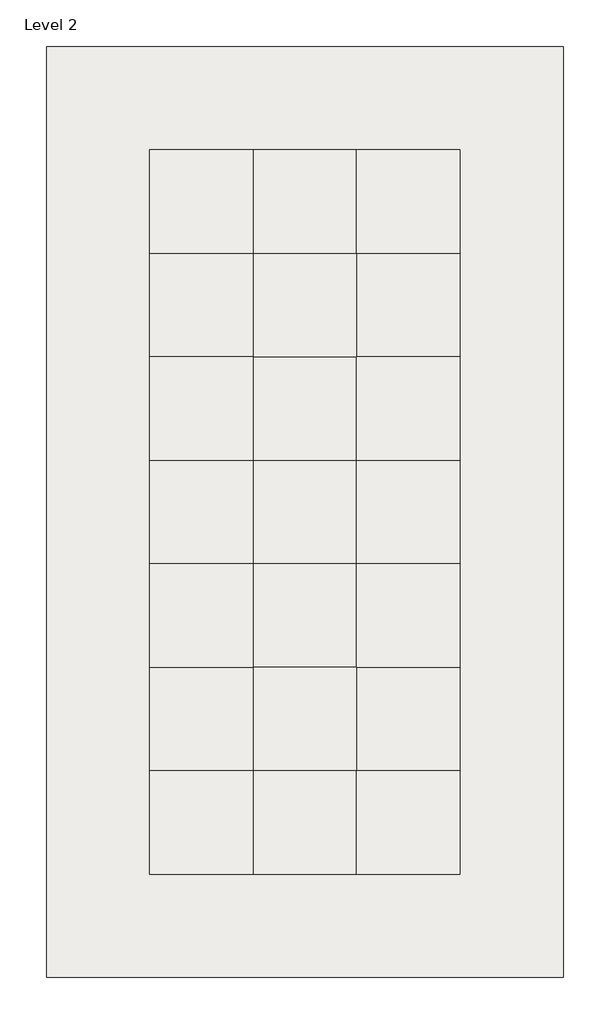
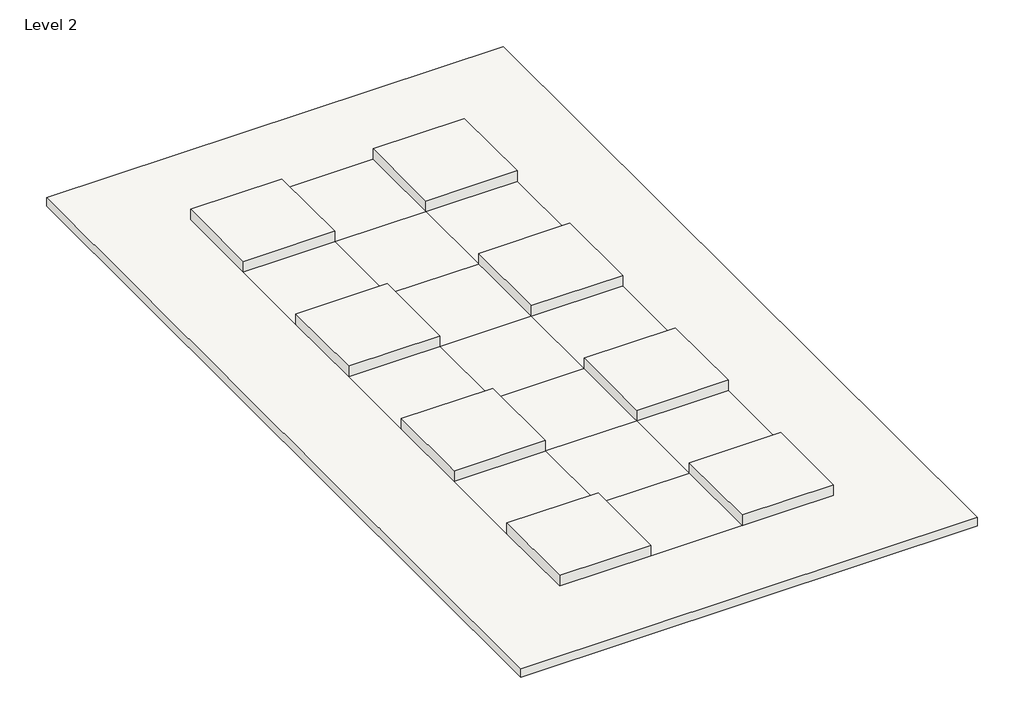
# One storey: 9 roofs.
"""IFC4 building model written with IfcOpenShell, lengths in millimetres."""

from ifc_helpers import new_model, si_unit, origin, place, context, project, spatial, faceted_brep, element, save

model = new_model("IFC4")

# Units and contexts
model_context = context("Model", 3, world=origin())
ifc_project = project(units=[si_unit("LENGTHUNIT", "METRE", prefix="MILLI")], contexts=[model_context])

# Site, building, storey
site = spatial("IfcSite", under=ifc_project)
building = spatial("IfcBuilding", under=site)
storey = spatial("IfcBuildingStorey", under=building, Name="Level 2", Elevation=8000.0)

# Roofs
placement = place(None, origin())
element("IfcRoof", 1, ObjectType="Bauder_RoofCoveringSystem_ExtensiveGreenRoofSystem_WildflowerBlanket", at=placement, inside=storey, context=model_context, shape_type="Brep", body=[
    faceted_brep([(-674.7340554, 1676.2074539, 8000.0), (1325.2659446, 1676.2074539, 8000.0), (1325.2659446, -323.7925461, 8000.0), (-674.7340554, -323.7925461, 8000.0), (1325.2659446, 1676.2074539, 8445.0), (-674.7340554, 1676.2074539, 8445.0), (-674.7340554, -323.7925461, 8445.0), (1325.2659446, -323.7925461, 8445.0), (1325.2659446, 1676.2074539, 8200.0), (-674.7340554, 1676.2074539, 8200.0), (-674.7340554, -323.7925461, 8200.0), (1325.2659446, -323.7925461, 8200.0)], [[[0, 1, 2, 3]], [[4, 5, 6, 7]], [[5, 4, 8, 1, 0, 9]], [[6, 5, 9, 0, 3, 10]], [[7, 6, 10, 3, 2, 11]], [[4, 7, 11, 2, 1, 8]]]),
])
element("IfcRoof", 2, ObjectType="Bauder_RoofCoveringSystem_ExtensiveGreenRoofSystem_WildflowerBlanket", at=placement, inside=storey, context=model_context, shape_type="Brep", body=[
    faceted_brep([(3325.2659446, 1676.2074539, 8000.0), (5325.2659446, 1676.2074539, 8000.0), (5325.2659446, -323.7925461, 8000.0), (3325.2659446, -323.7925461, 8000.0), (5325.2659446, 1676.2074539, 8445.0), (3325.2659446, 1676.2074539, 8445.0), (3325.2659446, -323.7925461, 8445.0), (5325.2659446, -323.7925461, 8445.0), (5325.2659446, 1676.2074539, 8200.0), (3325.2659446, 1676.2074539, 8200.0), (3325.2659446, -323.7925461, 8200.0), (5325.2659446, -323.7925461, 8200.0)], [[[0, 1, 2, 3]], [[4, 5, 6, 7]], [[5, 4, 8, 1, 0, 9]], [[6, 5, 9, 0, 3, 10]], [[7, 6, 10, 3, 2, 11]], [[4, 7, 11, 2, 1, 8]]]),
])
element("IfcRoof", 3, ObjectType="Bauder_RoofCoveringSystem_ExtensiveGreenRoofSystem_WildflowerBlanket", at=placement, inside=storey, context=model_context, shape_type="Brep", body=[
    faceted_brep([(3325.2659446, -2323.7925461, 8000.0), (5325.2659446, -2323.7925461, 8000.0), (5325.2659446, -4323.7925461, 8000.0), (3325.2659446, -4323.7925461, 8000.0), (5325.2659446, -2323.7925461, 8445.0), (3325.2659446, -2323.7925461, 8445.0), (3325.2659446, -4323.7925461, 8445.0), (5325.2659446, -4323.7925461, 8445.0), (5325.2659446, -2323.7925461, 8200.0), (3325.2659446, -2323.7925461, 8200.0), (3325.2659446, -4323.7925461, 8200.0), (5325.2659446, -4323.7925461, 8200.0)], [[[0, 1, 2, 3]], [[4, 5, 6, 7]], [[5, 4, 8, 1, 0, 9]], [[6, 5, 9, 0, 3, 10]], [[7, 6, 10, 3, 2, 11]], [[4, 7, 11, 2, 1, 8]]]),
])
element("IfcRoof", 4, ObjectType="Bauder_RoofCoveringSystem_ExtensiveGreenRoofSystem_WildflowerBlanket", at=placement, inside=storey, context=model_context, shape_type="Brep", body=[
    faceted_brep([(3325.2659446, -6323.7925461, 8000.0), (5325.2659446, -6323.7925461, 8000.0), (5325.2659446, -8323.7925461, 8000.0), (3325.2659446, -8323.7925461, 8000.0), (5325.2659446, -6323.7925461, 8445.0), (3325.2659446, -6323.7925461, 8445.0), (3325.2659446, -8323.7925461, 8445.0), (5325.2659446, -8323.7925461, 8445.0), (5325.2659446, -6323.7925461, 8200.0), (3325.2659446, -6323.7925461, 8200.0), (3325.2659446, -8323.7925461, 8200.0), (5325.2659446, -8323.7925461, 8200.0)], [[[0, 1, 2, 3]], [[4, 5, 6, 7]], [[5, 4, 8, 1, 0, 9]], [[6, 5, 9, 0, 3, 10]], [[7, 6, 10, 3, 2, 11]], [[4, 7, 11, 2, 1, 8]]]),
])
element("IfcRoof", 5, ObjectType="Bauder_RoofCoveringSystem_ExtensiveGreenRoofSystem_WildflowerBlanket", at=placement, inside=storey, context=model_context, shape_type="Brep", body=[
    faceted_brep([(3325.2659446, -10323.7925461, 8000.0), (5325.2659446, -10323.7925461, 8000.0), (5325.2659446, -12323.7925461, 8000.0), (3325.2659446, -12323.7925461, 8000.0), (5325.2659446, -10323.7925461, 8445.0), (3325.2659446, -10323.7925461, 8445.0), (3325.2659446, -12323.7925461, 8445.0), (5325.2659446, -12323.7925461, 8445.0), (5325.2659446, -10323.7925461, 8200.0), (3325.2659446, -10323.7925461, 8200.0), (3325.2659446, -12323.7925461, 8200.0), (5325.2659446, -12323.7925461, 8200.0)], [[[0, 1, 2, 3]], [[4, 5, 6, 7]], [[5, 4, 8, 1, 0, 9]], [[6, 5, 9, 0, 3, 10]], [[7, 6, 10, 3, 2, 11]], [[4, 7, 11, 2, 1, 8]]]),
])
element("IfcRoof", 6, ObjectType="Bauder_RoofCoveringSystem_ExtensiveGreenRoofSystem_WildflowerBlanket", at=placement, inside=storey, context=model_context, shape_type="Brep", body=[
    faceted_brep([(-674.7340554, -10323.7925461, 8000.0), (1325.2659446, -10323.7925461, 8000.0), (1325.2659446, -12323.7925461, 8000.0), (-674.7340554, -12323.7925461, 8000.0), (1325.2659446, -10323.7925461, 8445.0), (-674.7340554, -10323.7925461, 8445.0), (-674.7340554, -12323.7925461, 8445.0), (1325.2659446, -12323.7925461, 8445.0), (1325.2659446, -10323.7925461, 8200.0), (-674.7340554, -10323.7925461, 8200.0), (-674.7340554, -12323.7925461, 8200.0), (1325.2659446, -12323.7925461, 8200.0)], [[[0, 1, 2, 3]], [[4, 5, 6, 7]], [[5, 4, 8, 1, 0, 9]], [[6, 5, 9, 0, 3, 10]], [[7, 6, 10, 3, 2, 11]], [[4, 7, 11, 2, 1, 8]]]),
])
element("IfcRoof", 7, ObjectType="Bauder_RoofCoveringSystem_ExtensiveGreenRoofSystem_WildflowerBlanket", at=placement, inside=storey, context=model_context, shape_type="Brep", body=[
    faceted_brep([(-674.7340554, -6323.7925461, 8000.0), (1325.2659446, -6323.7925461, 8000.0), (1325.2659446, -8323.7925461, 8000.0), (-674.7340554, -8323.7925461, 8000.0), (1325.2659446, -6323.7925461, 8445.0), (-674.7340554, -6323.7925461, 8445.0), (-674.7340554, -8323.7925461, 8445.0), (1325.2659446, -8323.7925461, 8445.0), (1325.2659446, -6323.7925461, 8200.0), (-674.7340554, -6323.7925461, 8200.0), (-674.7340554, -8323.7925461, 8200.0), (1325.2659446, -8323.7925461, 8200.0)], [[[0, 1, 2, 3]], [[4, 5, 6, 7]], [[5, 4, 8, 1, 0, 9]], [[6, 5, 9, 0, 3, 10]], [[7, 6, 10, 3, 2, 11]], [[4, 7, 11, 2, 1, 8]]]),
])
element("IfcRoof", 8, ObjectType="Bauder_RoofCoveringSystem_ExtensiveGreenRoofSystem_WildflowerBlanket", at=placement, inside=storey, context=model_context, shape_type="Brep", body=[
    faceted_brep([(-674.7340554, -2323.7925461, 8000.0), (1325.2659446, -2323.7925461, 8000.0), (1325.2659446, -4323.7925461, 8000.0), (-674.7340554, -4323.7925461, 8000.0), (1325.2659446, -2323.7925461, 8445.0), (-674.7340554, -2323.7925461, 8445.0), (-674.7340554, -4323.7925461, 8445.0), (1325.2659446, -4323.7925461, 8445.0), (1325.2659446, -2323.7925461, 8200.0), (-674.7340554, -2323.7925461, 8200.0), (-674.7340554, -4323.7925461, 8200.0), (1325.2659446, -4323.7925461, 8200.0)], [[[0, 1, 2, 3]], [[4, 5, 6, 7]], [[5, 4, 8, 1, 0, 9]], [[6, 5, 9, 0, 3, 10]], [[7, 6, 10, 3, 2, 11]], [[4, 7, 11, 2, 1, 8]]]),
])
element("IfcRoof", 9, ObjectType="Roof_Concrete-200mm", at=placement, inside=storey, context=model_context, shape_type="Brep", body=[
    faceted_brep([(-2674.7340554, -14323.7925461, 8200.0), (-2674.7340554, -14323.7925461, 8000.0), (7325.2659446, -14323.7925461, 8000.0), (7325.2659446, -14323.7925461, 8200.0), (-2674.7340554, 3676.2074539, 8200.0), (-2674.7340554, 3676.2074539, 8000.0), (7325.2659446, 3676.2074539, 8200.0), (7325.2659446, 3676.2074539, 8000.0), (3325.2659446, 1676.2074539, 8200.0), (1325.2659446, 1676.2074539, 8200.0), (1325.2659446, -323.7925461, 8200.0), (3325.2659446, -323.7925461, 8200.0), (1325.2659446, 1676.2074539, 8000.0), (3325.2659446, 1676.2074539, 8000.0), (3325.2659446, -323.7925461, 8000.0), (1325.2659446, -323.7925461, 8000.0), (1325.2659446, -2323.7925461, 8200.0), (-674.7340554, -323.7925461, 8200.0), (-674.7340554, -2323.7925461, 8200.0), (3325.2659446, -2323.7925461, 8200.0), (5325.2659446, -2323.7925461, 8200.0), (5325.2659446, -323.7925461, 8200.0), (-674.7340554, -2323.7925461, 8000.0), (-674.7340554, -323.7925461, 8000.0), (1325.2659446, -2323.7925461, 8000.0), (3325.2659446, -2323.7925461, 8000.0), (5325.2659446, -323.7925461, 8000.0), (5325.2659446, -2323.7925461, 8000.0), (1325.2659446, -4323.7925461, 8200.0), (3325.2659446, -4323.7925461, 8200.0), (3325.2659446, -4323.7925461, 8000.0), (1325.2659446, -4323.7925461, 8000.0), (1325.2659446, -6323.7925461, 8200.0), (-674.7340554, -4323.7925461, 8200.0), (-674.7340554, -6323.7925461, 8200.0), (5325.2659446, -6323.7925461, 8200.0), (5325.2659446, -4323.7925461, 8200.0), (3325.2659446, -6323.7925461, 8200.0), (-674.7340554, -6323.7925461, 8000.0), (-674.7340554, -4323.7925461, 8000.0), (1325.2659446, -6323.7925461, 8000.0), (3325.2659446, -6323.7925461, 8000.0), (5325.2659446, -4323.7925461, 8000.0), (5325.2659446, -6323.7925461, 8000.0), (1325.2659446, -12323.7925461, 8200.0), (3325.2659446, -12323.7925461, 8200.0), (3325.2659446, -10323.7925461, 8200.0), (1325.2659446, -10323.7925461, 8200.0), (3325.2659446, -12323.7925461, 8000.0), (1325.2659446, -12323.7925461, 8000.0), (1325.2659446, -10323.7925461, 8000.0), (3325.2659446, -10323.7925461, 8000.0), (1325.2659446, -8323.7925461, 8200.0), (-674.7340554, -8323.7925461, 8200.0), (-674.7340554, -10323.7925461, 8200.0), (3325.2659446, -8323.7925461, 8200.0), (5325.2659446, -10323.7925461, 8200.0), (5325.2659446, -8323.7925461, 8200.0), (-674.7340554, -10323.7925461, 8000.0), (-674.7340554, -8323.7925461, 8000.0), (1325.2659446, -8323.7925461, 8000.0), (3325.2659446, -8323.7925461, 8000.0), (5325.2659446, -8323.7925461, 8000.0), (5325.2659446, -10323.7925461, 8000.0), (-674.7340554, 1676.2074539, 8000.0), (-674.7340554, 1676.2074539, 8200.0), (5325.2659446, 1676.2074539, 8200.0), (5325.2659446, 1676.2074539, 8000.0), (5325.2659446, -12323.7925461, 8000.0), (5325.2659446, -12323.7925461, 8200.0), (-674.7340554, -12323.7925461, 8000.0), (-674.7340554, -12323.7925461, 8200.0)], [[[0, 1, 2, 3]], [[1, 0, 4, 5]], [[6, 7, 5, 4]], [[3, 2, 7, 6]], [[8, 9, 10, 11]], [[12, 13, 14, 15]], [[16, 10, 17, 18]], [[11, 10, 16, 19]], [[20, 21, 11, 19]], [[22, 23, 15, 24]], [[15, 14, 25, 24]], [[25, 14, 26, 27]], [[19, 16, 28, 29]], [[24, 25, 30, 31]], [[32, 28, 33, 34]], [[35, 36, 29, 37]], [[38, 39, 31, 40]], [[41, 30, 42, 43]], [[44, 45, 46, 47]], [[48, 49, 50, 51]], [[47, 52, 53, 54]], [[47, 46, 55, 52]], [[56, 57, 55, 46]], [[58, 59, 60, 50]], [[51, 50, 60, 61]], [[51, 61, 62, 63]], [[52, 55, 37, 32]], [[29, 28, 32, 37]], [[61, 60, 40, 41]], [[31, 30, 41, 40]], [[9, 12, 15, 10]], [[10, 15, 23, 17]], [[17, 23, 64, 65]], [[12, 9, 65, 64]], [[66, 67, 26, 21]], [[21, 26, 14, 11]], [[11, 14, 13, 8]], [[67, 66, 8, 13]], [[20, 27, 42, 36]], [[36, 42, 30, 29]], [[29, 30, 25, 19]], [[27, 20, 19, 25]], [[16, 24, 31, 28]], [[28, 31, 39, 33]], [[33, 39, 22, 18]], [[24, 16, 18, 22]], [[32, 40, 60, 52]], [[52, 60, 59, 53]], [[53, 59, 38, 34]], [[40, 32, 34, 38]], [[35, 43, 62, 57]], [[57, 62, 61, 55]], [[55, 61, 41, 37]], [[43, 35, 37, 41]], [[56, 63, 68, 69]], [[69, 68, 48, 45]], [[45, 48, 51, 46]], [[63, 56, 46, 51]], [[47, 50, 49, 44]], [[44, 49, 70, 71]], [[71, 70, 58, 54]], [[50, 47, 54, 58]], [[4, 0, 3, 6], [9, 8, 66, 21, 20, 36, 35, 57, 56, 69, 45, 44, 71, 54, 53, 34, 33, 18, 17, 65]], [[7, 2, 1, 5], [13, 12, 64, 23, 22, 39, 38, 59, 58, 70, 49, 48, 68, 63, 62, 43, 42, 27, 26, 67]]]),
])

save(model, "model.ifc")

# Revit data of these elements
# Type "Bauder_RoofCoveringSystem_ExtensiveGreenRoofSystem_WildflowerBlanket"
#   Keynote = "Q37"
#   Type IFC Predefined Type = "FLAT_ROOF"
#   Export Type to IFC As = "IfcRoofType"
#   Model = "Bauder Biodiverse Wildflower Blanket - Extensive Green Roof System"
#   Manufacturer = "Bauder Ltd"
#   Type Comments = "Wildflower Blanket"
#   URL = "https://www.bauder.co.uk/"
#   Description = "Bauder Biodiverse GreenRoof system incorporating WB 25 mm UK Native Species Wildflower Blanket with Biodiverse Substrate, Filter Fleece, DSE40 Polyethylene Drainage and Protection Layer, and FSM600 Polyester-Polypropylene fibre protection mat."
#   Assembly Code = "B3010"
#   NBSDescription = "Extensive green roof system"
#   NBSReference = "45-40-47/130"
#   BIMObjectName = "Bauder_RoofCoveringSystem_ExtensiveGreenRoofSystem_WildflowerBlanket"
#   AccessibilityPerformance = "n/a"
#   CodePerformance = "n/a"
#   Color = "n/a"
#   Constituents = "n/a"
#   DurationUnit = "Year"
#   ExpectedLife = "n/a"
#   Features = "This BIM Object must be supported by a project specific specification from Bauder, incorporating system build-up, detail design and performance calculations if a full Bauder system guarantee is required. Please contact your local Bauder Representative or technical@bauder.co.uk"
#   Finish = "n/a"
#   Grade = "n/a"
#   Material = "n/a"
#   ModelReference = "Bauder Biodiverse Wildflower Blanket - Extensive Green Roof System"
#   Name = "RoofCoveringSystem_Bauder_ExtensiveGreenRoofSystem"
#   ReplacementCost = "n/a"
#   Shape = "n/a"
#   Size = "n/a"
#   SustainabilityPerformance = "Bauder Germany ISO14001: Certificate No.: 70499/03-15 e, Bauder UK ISO14001:Certificate No. 19ACM6595R, EN1271, BREEAM Credits Available"
#   WarrantyDescription = "Guarantee options could include ‘Product’, ‘Product and Workmanship’ and ‘Product, Workmanship and Design’ Guarantees. All guarantees available for this system are subject to the works being carried out in accordance with the Bauder specification and being installed by a Bauder Approved installer. For full details and further information regarding guarantees and alternative systems please contact your local Bauder Representative or technical@bauder.co.uk"
#   WarrantyDurationLabor = "n/a"
#   WarrantyDurationParts = "n/a"
#   WarrantyDurationUnit = "Year"
#   WarrantyGuarantorLabor = "n/a"
#   WarrantyGuarantorParts = "technical@bauder.co.uk"
#   Certification = "Comply with GRO Green Roof Code of Practice and FLL Standards"
#   EdgeRestraints = "Perforated edge trim where required, refer to Bauder Project Specific Specification"
#   MoistureControlDrainageAncillaries = "n/a"
#   MoistureControlDrainageLayer = "Bauder DSE40 40 mm Polyethylene Drainage and Protection Layer"
#   MoistureControlFilterMembrane = "Bauder Filter Fleece 1 mm Polypropylene Filter Fleece"
#   MoistureControlMoistureRetentionMat = "Polypropylene mesh bonded to a moisture permeable base carrier sheet integral to the Blanket"
#   PlantingSystemsAntierosionMat = "Jute Net where exposed, refer to Bauder Project Specific Specification"
#   PlantingSystemsPlantingMedium = "Bauder Biodiverse Substrate Recycled crushed brick, expanded clay shale and composted pine bark"
#   PlantingSystemsVegetation = "Bauder WB 25 mm UK Native Species Wildflower Blanket"
#   PlantingSystemsVegetationBarrier = "20-40 mm Rounded-Washed Stones, refer to Bauder Project Specific Specification"
#   ProjectSpecificationAndDesign = "This BIM Object must be supported by a project specific specification from Bauder, incorporating system build-up, detail design and performance calculations if a full Bauder system warranty is required. Please contact your local Bauder Representative or technical@bauder.co.uk"
#   ProtectionProtectionLayer = "Bauder FSM600 4 mm Polyester-Polypropylene fibre protection mat"
#   ProtectionRootBarrier = "As per project specific Bauder Specification"
#   ProtectionSeparationLayer = "n/a"
#   SystemManufacturer = "Bauder Ltd"
#   WarrantyConsiderations = "All guarantees available for this system are subject to the works being carried out in accordance with the Bauder specification and being installed by a Bauder Approved installer. For full details and further information regarding guarantees and alternative systems please contact your local Bauder Representative or technical@bauder.co.uk"
#   Update = "1900-12-31T23:59:59"
#   Documentation = "https://www.bauder.co.uk/technical-centre/technical-literature/system-brochures"
#   DocumentReference = "http://www.bauder.co.uk/"
#   IfcExportAs = "IfcRoofType"
#   IfcExportType = "FLAT_ROOF"
#   MethodOfMesurement = "n/a"
#   Process = "Replacement at service life intervals"
#   FireRating = "n/a"
#   _Author = "AM"
#   _AuthorizedBy = "bimstore"
#   _CreatedBy = "technical@bauder.co.uk"
#   _DistributedBy = "www.bimstore.co"
#   AssetType = "Fixed"
#   ClassificationName = "Uniclass2015"
#   ClassificationValue = "Ss_45_40_47_09"
#   CreatedBy = "technical@bauder.co.uk"
#   CreatedOn = "2023-02-10 T00:00:00"
#   DocumentationCertificates = "n/a"
#   DocumentationInstallationGuide = "https://www.bauder.co.uk/technical-centre"
#   DocumentationLiterature = "https://www.bauder.co.uk/technical-centre"
#   DocumentationMaintenance = "https://www.bauder.co.uk/technical-centre/maintenance-advice"
#   DocumentationTechnical = "https://www.bauder.co.uk/green-roofs/extensive-green-roofs/biodiverse-or-brown-roofs/wildflower-blanket"
#   ManufacturerName = "Bauder Ltd"
#   ModelNumber = "0905_WB-BioS-FF-D4-F6"
#   ProductionYear = "2017"
#   ReferencedStandard = "n/a"
#   SpareParts = "n/a"
#   TypeName = "Wildflower Blanket"
#   NBSNote = "n/a"
#   NBSObjectName = "Bauder - Extensive green roof system"
#   NBSOfficeMasterTag = "n/a"
#   Ballast = "n/a"
#   CarrierMembraneFixing = "n/a"
#   CarrierMembraneType = "n/a"
#   FillToPerimeterUpstands = "n/a"
#   FilterLayer = "n/a"
#   InsulationFixing = "n/a"
#   InsulationType = "n/a"
#   LiquidAppliedWaterproofCoatingReinforcement = "n/a"
#   LiquidAppliedWaterproofCoatingSurfaceTreatment = "n/a"
#   LiquidAppliedWaterproofCoatingType = "n/a"
#   PreparationExistingSubstrates = "n/a"
#   PreparationHorizontalWork = "n/a"
#   PreparationSkirtingsAndVerticalWork = "n/a"
#   ProtectionLayer = "n/a"
#   SystemAccessories = "n/a"
#   WaterproofCoveringFirstLayerAttachment = "n/a"
#   WaterproofCoveringFirstLayerType = "n/a"
#   WaterproofCoveringIntermediateLayerAttachment = "n/a"
#   WaterproofCoveringIntermediateLayerType = "n/a"
#   WaterproofCoveringTopLayerAttachment = "n/a"
#   InsulationAttachment = "n/a"
#   IsolatingLayer = "n/a"
#   CarrierMembraneAttachment = "n/a"
#   LiquidAppliedWaterproofCoatingWearingCourse = "n/a"
#   VapourControlLayer = "n/a"
#   VapourControlLayerAttachment_Bauder = "n/a"
#   WaterproofCoveringJoints = "n/a"
#   WaterproofCoveringType = "n/a"
#   SeparatingLayer = "n/a"
#   WaterproofCoveringAccessories = "Yes"
#   WaterproofCoveringAttachment = "n/a"
#   UpperProtectionLayer = "n/a"
#   LowerProtectionLayer = "n/a"
#   WaterproofCoveringTopLayerType = "n/a"
#   DetailWorkAncillaryItems = "Detail as per project specific Bauder Specification"
#   DetailWorkCoverStrips = "Detail as per project specific Bauder Specification"
#   DetailWorkFlashings = "Detail as per project specific Bauder Specification"
#   DetailWorkSkirtingsAndUpstands = "Detail as per project specific Bauder Specification"
#   DetailWorkWeltedDrips = "Detail as per project specific Bauder Specification"
#   OverlayFixing = "n/a"
#   OverlayType = "n/a"
#   SurfaceProtection = "n/a"
#   VapourControlLayerAttachment = "n/a"
#   VapourControlLayerType = "n/a"
#   Cost = 0
#   NominalHeight = 0 mm
#   NominalLength = 0 mm
#   TotalArea = 0 m²
#   NominalDepth = 0 mm
#   IsExternal = yes
#   _BimSpecGuid = 0
#   _BSBibleVersion = 16
#   _CurrentRevision = 4
#   Layers, outside or top first: 100 mm "Bauder_Vegetation_BauderGREEN-WB-Wildflower-Blanket" (function 5); 100 mm "Bauder_ExtensiveSubstrate_BauderGREEN-SUB-BM-UK" (function 2); 1 mm "Bauder_FilterFleece_BauderGREEN-FV-125-100" (function 3); 40 mm "Bauder_DrainageBoard_BauderGREEN-DSE-40" (function 3); 4 mm "Bauder_ProtectionMat_BauderGREEN-FSM-600" (function 3); 200 mm "Concrete" (function 1)
# Type "Roof_Concrete-200mm"
#   Layers, outside or top first: 200 mm "Concrete" (function 1)
# Elements 1, 2, 3, 4, 5, 6, 7, 8 (IfcRoof, "Bauder_RoofCoveringSystem_ExtensiveGreenRoofSystem_WildflowerBlanket")
#   built-in parameter 1001705 = 27.7067 (stored number, unit not read)
#   built-in parameter 1001710 = 33615
#   Phase Created = New Construction
#   Materials on its faces: "Concrete", "Bauder_Vegetation_BauderGREEN-WB-Wildflower-Blanket"
# Element 9 (IfcRoof, "Roof_Concrete-200mm")
#   built-in parameter 1001710 = 33615
#   Phase Created = New Construction
#   Materials on its faces: "Concrete"
# Materials
#   "Bauder_Vegetation_BauderGREEN-WB-Wildflower-Blanket": class "Unassigned", colour RGB 71 83 38, transparency 0, Mtrl_Author = "AM", Mtrl_AuthorizedBy = "bimstore", Mtrl_DistributedBy = "www.bimstore.co", Mtrl_AccessibilityPerformance = "n/a", Mtrl_AssetIdentifier = "Please record on commissioning", Mtrl_AssetType = "Fixed", Mtrl_BarCode = "Please record on commissioning", Mtrl_ClassificationName = "Uniclass2020", Mtrl_ClassificationValue = "Ss_45_40_47_09", Mtrl_CodePerformance = "n/a", Mtrl_Color = "n/a", Mtrl_Constituents = "n/a", Mtrl_CreatedBy = "technical@bauder.co.uk", Mtrl_CreatedOn = "2023-02-10 T00:00:00", Mtrl_DocumentationCertificates = "https://www.bimstore.co/products/extensive-green-roof-system-wildflower-blanket/document/product-certificates", Mtrl_DocumentationInstallationGuide = "https://www.bimstore.co/products/extensive-green-roof-system-wildflower-blanket/document/installation-guide", Mtrl_DocumentationLiterature = "https://www.bimstore.co/products/extensive-green-roof-system-wildflower-blanket/document/product-literature", Mtrl_DocumentationMaintenance = "https://www.bimstore.co/products/extensive-green-roof-system-wildflower-blanket/document/maintenance-information", Mtrl_DocumentationTechnical = "https://www.bimstore.co/products/extensive-green-roof-system-wildflower-blanket/document/technical-data-sheet", Mtrl_DurationUnit = "Year", Mtrl_Features = "n/a", Mtrl_Finish = "n/a", Mtrl_Grade = "n/a", Mtrl_InstallationDate = "Please record on commissioning", Mtrl_ManufacturerName = "Bauder Ltd", Mtrl_Material = "Substrate and wildflower plants, embedded in a nylon mesh, with a moisture retention fleece", Mtrl_ModelNumber = "BauderGREEN-WB-Wildflower-Blanket", Mtrl_ModelReference = "Vegetation", Mtrl_ProductionYear = "2023", Mtrl_ReferencedStandard = "n/a", Mtrl_Shape = "n/a", Mtrl_Size = "n/a", Mtrl_SpareParts = "n/a", Mtrl_TypeName = "BauderGREEN-WB-Wildflower-Blanket", Mtrl_WarrantyDescription = "As part of Bauder system guarantee, per specification", Mtrl_WarrantyDurationUnit = "Year", Mtrl_WarrantyGuarantorLabor = "technical@bauder.co.uk", Mtrl_WarrantyGuarantorParts = "technical@bauder.co.uk", Mtrl_WarrantyStartDate = "Please record on commissioning", Mtrl_IfcExportAs = "IfcRoofType", Mtrl_IfcExportType = "FLAT_ROOF", Mtrl_BIMObjectName = "Bauder_Vegetation_BauderGREEN-WB-Wildflower-Blanket", Mtrl_NBSDescription = "n/a", Mtrl_NBSNote = "n/a", Mtrl_NBSObjectName = "n/a", Mtrl_NBSOfficeMasterTag = "n/a", Mtrl_NBSReference = "Q37", Mtrl_Ballast = "n/a", Mtrl_CarrierMembraneAttachment = "n/a", Mtrl_CarrierMembraneFixing = "n/a", Mtrl_CarrierMembraneType = "n/a", Mtrl_Certification = "Comply with GRO Green Roof Code of Practice and FLL Standards", Mtrl_DetailWorkAncillaryItems = "Detail as per project specific Bauder Specification", Mtrl_DetailWorkCoverStrips = "Detail as per project specific Bauder Specification", Mtrl_DetailWorkFlashings = "Detail as per project specific Bauder Specification", Mtrl_DetailWorkSkirtingsAndUpstands = "Detail as per project specific Bauder Specification", Mtrl_DetailWorkWeltedDrips = "Detail as per project specific Bauder Specification", Mtrl_EdgeRestraints = "Detail as per project specific Bauder Specification", Mtrl_FillToPerimeterUpstands = "n/a", Mtrl_FilterLayer = "n/a", Mtrl_InsulationAttachment = "As per project specific Bauder Specification", Mtrl_InsulationFixing = "As per project specific Bauder Specification", Mtrl_InsulationType = "As per project specific Bauder Specification", Mtrl_IsolatingLayer = "n/a", Mtrl_LiquidAppliedWaterproofCoatingReinforcement = "As per project specific Bauder Specification", Mtrl_LiquidAppliedWaterproofCoatingSurfaceTreatment = "As per project specific Bauder Specification", Mtrl_LiquidAppliedWaterproofCoatingType = "As per project specific Bauder Specification", Mtrl_LiquidAppliedWaterproofCoatingWearingCourse = "As per project specific Bauder Specification", Mtrl_LowerProtectionLayer = "n/a", Mtrl_MoistureControlDrainageAncillaries = "n/a", Mtrl_MoistureControlDrainageLayer = "n/a", Mtrl_MoistureControlFilterMembrane = "n/a", Mtrl_MoistureControlMoistureRetentionMat = "n/a", Mtrl_OverlayFixing = "n/a", Mtrl_OverlayType = "n/a", Mtrl_PlantingSystemsAntierosionMat = "n/a", Mtrl_PlantingSystemsPlantingMedium = "As per project specific Bauder Specification", Mtrl_PlantingSystemsVegetation = "As per project specific Bauder Specification", Mtrl_PlantingSystemsVegetationBarrier = "As per project specific Bauder Specification", Mtrl_PreparationExistingSubstrates = "n/a", Mtrl_PreparationHorizontalWork = "n/a", Mtrl_PreparationSkirtingsAndVerticalWork = "n/a", Mtrl_ProjectSpecificationAndDesign = "This BIM Object must be supported by a project specific specification from Bauder, incorporating system build-up, detail design and performance calculations if a full Bauder system warranty is required. Please contact your local Bauder Representative or technical@bauder.co.uk", Mtrl_ProtectionLayer = "n/a", Mtrl_ProtectionProtectionLayer = "n/a", Mtrl_ProtectionRootBarrier = "As per project specific Bauder Specification", Mtrl_ProtectionSeparationLayer = "n/a", Mtrl_SeparatingLayer = "n/a", Mtrl_SurfaceProtection = "n/a", Mtrl_SystemAccessories = "n/a", Mtrl_SystemManufacturer = "Bauder Ltd", Mtrl_Update = "1900-12-31 T23:59:59", Mtrl_UpperProtectionLayer = "n/a", Mtrl_VapourControlLayerAttachment = "As per project specific Bauder Specification", Mtrl_VapourControlLayerAttachment_Bauder = "As per project specific Bauder Specification", Mtrl_VapourControlLayerType = "As per project specific Bauder Specification", Mtrl_WarrantyConsiderations = "All guarantees available for this system are subject to the works being carried out in accordance with the Bauder specification and being installed by a Bauder Approved installer. For full details and further information regarding guarantees and alternative systems please contact your local Bauder Representative or technical@bauder.co.uk", Mtrl_WaterproofCoveringAccessories = "As per project specific Bauder Specification", Mtrl_WaterproofCoveringAttachment = "As per project specific Bauder Specification", Mtrl_WaterproofCoveringFirstLayerAttachment = "As per project specific Bauder Specification", Mtrl_WaterproofCoveringFirstLayerType = "As per project specific Bauder Specification", Mtrl_WaterproofCoveringIntermediateLayerAttachment = "As per project specific Bauder Specification", Mtrl_WaterproofCoveringIntermediateLayerType = "As per project specific Bauder Specification", Mtrl_WaterproofCoveringJoints = "As per project specific Bauder Specification", Mtrl_WaterproofCoveringTopLayerAttachment = "As per project specific Bauder Specification", Mtrl_WaterproofCoveringTopLayerType = "As per project specific Bauder Specification", Mtrl_WaterproofCoveringType = "As per project specific Bauder Specification", Cost = 0, Mtrl_ReplacementCost = 0, Mtrl_NominalDepth = 30 mm, Mtrl_NominalHeight = 0 mm, Mtrl_NominalLength = 0 mm, Mtrl_BimSpecGuid = 0, Mtrl_BSBibleVersion = 17, Mtrl_CurrentRevision = 2, Mtrl_ExpectedLife = 0, Mtrl_SerialNumber = 0, Mtrl_WarrantyDurationLabor = 0, Mtrl_WarrantyDurationParts = 0
#   "Bauder_ExtensiveSubstrate_BauderGREEN-SUB-BM-UK": class "Unassigned", colour RGB 255 255 255, transparency 0, Mtrl_Author = "AM", Mtrl_AuthorizedBy = "bimstore", Mtrl_DistributedBy = "www.bimstore.co", Mtrl_AccessibilityPerformance = "n/a", Mtrl_AssetIdentifier = "Please record on commissioning", Mtrl_AssetType = "Fixed", Mtrl_BarCode = "Please record on commissioning", Mtrl_ClassificationName = "Uniclass2019", Mtrl_ClassificationValue = "n/a", Mtrl_CodePerformance = "n/a", Mtrl_Color = "n/a", Mtrl_Constituents = "n/a", Mtrl_CreatedBy = "technical@bauder.co.uk", Mtrl_CreatedOn = "2023-02-10 T00:00:00", Mtrl_DocumentationCertificates = "https://www.bimstore.co/products/extensive-green-roof-system-wildflower-blanket/document/product-certificates", Mtrl_DocumentationInstallationGuide = "https://www.bimstore.co/products/extensive-green-roof-system-wildflower-blanket/document/installation-guide", Mtrl_DocumentationLiterature = "https://www.bimstore.co/products/extensive-green-roof-system-wildflower-blanket/document/product-literature", Mtrl_DocumentationMaintenance = "https://www.bimstore.co/products/extensive-green-roof-system-wildflower-blanket/document/maintenance-information", Mtrl_DocumentationTechnical = "https://www.bimstore.co/products/extensive-green-roof-system-wildflower-blanket/document/technical-data-sheet", Mtrl_DurationUnit = "Year", Mtrl_Features = "n/a", Mtrl_Finish = "n/a", Mtrl_Grade = "n/a", Mtrl_InstallationDate = "Please record on commissioning", Mtrl_ManufacturerName = "Bauder Ltd", Mtrl_Material = "Recycled crushed brick, expanded clay, shale, composted pine bark", Mtrl_ModelNumber = "BauderGREEN-SUB-BM-UK", Mtrl_ModelReference = "Extensive Substrate", Mtrl_ProductionYear = "2023", Mtrl_ReferencedStandard = "n/a", Mtrl_Shape = "n/a", Mtrl_Size = "n/a", Mtrl_SpareParts = "n/a", Mtrl_TypeName = "BauderGREEN-SUB-BM-UK", Mtrl_WarrantyDescription = "As part of Bauder system guarantee, per specification", Mtrl_WarrantyDurationUnit = "Year", Mtrl_WarrantyGuarantorLabor = "technical@bauder.co.uk", Mtrl_WarrantyGuarantorParts = "technical@bauder.co.uk", Mtrl_WarrantyStartDate = "Please record on commissioning", Mtrl_IfcExportAs = "IfcRoofType", Mtrl_IfcExportType = "FLAT_ROOF", Mtrl_BIMObjectName = "Bauder_ExtensiveSubstrate_BauderGREEN-SUB-BM-UK", Mtrl_NBSDescription = "n/a", Mtrl_NBSNote = "n/a", Mtrl_NBSObjectName = "n/a", Mtrl_NBSOfficeMasterTag = "n/a", Mtrl_NBSReference = "Q37", Mtrl_Ballast = "n/a", Mtrl_CarrierMembraneAttachment = "n/a", Mtrl_CarrierMembraneFixing = "n/a", Mtrl_CarrierMembraneType = "n/a", Mtrl_Certification = "Comply with GRO Green Roof Code of Practice and FLL Standards", Mtrl_DetailWorkAncillaryItems = "Detail as per project specific Bauder Specification", Mtrl_DetailWorkCoverStrips = "Detail as per project specific Bauder Specification", Mtrl_DetailWorkFlashings = "Detail as per project specific Bauder Specification", Mtrl_DetailWorkSkirtingsAndUpstands = "Detail as per project specific Bauder Specification", Mtrl_DetailWorkWeltedDrips = "Detail as per project specific Bauder Specification", Mtrl_EdgeRestraints = "Detail as per project specific Bauder Specification", Mtrl_FillToPerimeterUpstands = "n/a", Mtrl_FilterLayer = "n/a", Mtrl_InsulationAttachment = "As per project specific Bauder Specification", Mtrl_InsulationFixing = "As per project specific Bauder Specification", Mtrl_InsulationType = "As per project specific Bauder Specification", Mtrl_IsolatingLayer = "n/a", Mtrl_LiquidAppliedWaterproofCoatingReinforcement = "As per project specific Bauder Specification", Mtrl_LiquidAppliedWaterproofCoatingSurfaceTreatment = "As per project specific Bauder Specification", Mtrl_LiquidAppliedWaterproofCoatingType = "As per project specific Bauder Specification", Mtrl_LiquidAppliedWaterproofCoatingWearingCourse = "As per project specific Bauder Specification", Mtrl_LowerProtectionLayer = "As per project specific Bauder Specification", Mtrl_MoistureControlDrainageAncillaries = "n/a", Mtrl_MoistureControlDrainageLayer = "n/a", Mtrl_MoistureControlFilterMembrane = "n/a", Mtrl_MoistureControlMoistureRetentionMat = "n/a", Mtrl_OverlayFixing = "n/a", Mtrl_OverlayType = "n/a", Mtrl_PlantingSystemsAntierosionMat = "n/a", Mtrl_PlantingSystemsPlantingMedium = "As per project specific Bauder Specification", Mtrl_PlantingSystemsVegetation = "As per project specific Bauder Specification", Mtrl_PlantingSystemsVegetationBarrier = "As per project specific Bauder Specification", Mtrl_PreparationExistingSubstrates = "n/a", Mtrl_PreparationHorizontalWork = "n/a", Mtrl_PreparationSkirtingsAndVerticalWork = "n/a", Mtrl_ProjectSpecificationAndDesign = "This BIM Object must be supported by a project specific specification from Bauder, incorporating system build-up, detail design and performance calculations if a full Bauder system warranty is required. Please contact your local Bauder Representative or technical@bauder.co.uk", Mtrl_ProtectionLayer = "n/a", Mtrl_ProtectionProtectionLayer = "n/a", Mtrl_ProtectionRootBarrier = "As per project specific Bauder Specification", Mtrl_ProtectionSeparationLayer = "n/a", Mtrl_SeparatingLayer = "n/a", Mtrl_SurfaceProtection = "n/a", Mtrl_SystemAccessories = "n/a", Mtrl_SystemManufacturer = "Bauder Ltd", Mtrl_Update = "1900-12-31 T23:59:59", Mtrl_UpperProtectionLayer = "n/a", Mtrl_VapourControlLayerAttachment = "As per project specific Bauder Specification", Mtrl_VapourControlLayerAttachment_Bauder = "As per project specific Bauder Specification", Mtrl_VapourControlLayerType = "As per project specific Bauder Specification", Mtrl_WarrantyConsiderations = "All guarantees available for this system are subject to the works being carried out in accordance with the Bauder specification and being installed by a Bauder Approved installer. For full details and further information regarding guarantees and alternative systems please contact your local Bauder Representative or technical@bauder.co.uk", Mtrl_WaterproofCoveringAccessories = "As per project specific Bauder Specification", Mtrl_WaterproofCoveringAttachment = "As per project specific Bauder Specification", Mtrl_WaterproofCoveringFirstLayerAttachment = "As per project specific Bauder Specification", Mtrl_WaterproofCoveringFirstLayerType = "As per project specific Bauder Specification", Mtrl_WaterproofCoveringIntermediateLayerAttachment = "As per project specific Bauder Specification", Mtrl_WaterproofCoveringIntermediateLayerType = "As per project specific Bauder Specification", Mtrl_WaterproofCoveringJoints = "As per project specific Bauder Specification", Mtrl_WaterproofCoveringTopLayerAttachment = "As per project specific Bauder Specification", Mtrl_WaterproofCoveringTopLayerType = "As per project specific Bauder Specification", Mtrl_WaterproofCoveringType = "As per project specific Bauder Specification", Cost = 0, Mtrl_ReplacementCost = 0, Mtrl_NominalDepth = 100 mm, Mtrl_NominalHeight = 0 mm, Mtrl_NominalLength = 0 mm, Mtrl_BimSpecGuid = 0, Mtrl_BSBibleVersion = 17, Mtrl_CurrentRevision = 2, Mtrl_ExpectedLife = 0, Mtrl_SerialNumber = 0, Mtrl_WarrantyDurationLabor = 0, Mtrl_WarrantyDurationParts = 0
#   "Bauder_FilterFleece_BauderGREEN-FV-125-100": class "Unassigned", colour RGB 255 255 255, transparency 0, Mtrl_Author = "AM", Mtrl_AuthorizedBy = "bimstore", Mtrl_DistributedBy = "www.bimstore.co", Mtrl_AccessibilityPerformance = "n/a", Mtrl_AssetIdentifier = "Please record on commissioning", Mtrl_AssetType = "Fixed", Mtrl_BarCode = "Please record on commissioning", Mtrl_ClassificationName = "Uniclass2015", Mtrl_ClassificationValue = "n/a", Mtrl_CodePerformance = "n/a", Mtrl_Color = "n/a", Mtrl_Constituents = "n/a", Mtrl_CreatedBy = "technical@bauder.co.uk", Mtrl_CreatedOn = "2023-02-10 T00:00:00", Mtrl_DocumentationCertificates = "https://www.bimstore.co/products/extensive-green-roof-system-wildflower-blanket/document/product-certificates", Mtrl_DocumentationInstallationGuide = "https://www.bimstore.co/products/extensive-green-roof-system-wildflower-blanket/document/installation-guide", Mtrl_DocumentationLiterature = "https://www.bimstore.co/products/intensive-green-roof-system/document/product-literature", Mtrl_DocumentationMaintenance = "https://www.bimstore.co/products/extensive-green-roof-system-wildflower-blanket/document/maintenance-information", Mtrl_DocumentationTechnical = "https://www.bimstore.co/products/extensive-green-roof-system-wildflower-blanket/document/technical-data-sheet", Mtrl_DurationUnit = "Year", Mtrl_Features = "n/a", Mtrl_Finish = "n/a", Mtrl_Grade = "n/a", Mtrl_InstallationDate = "Please record on commissioning", Mtrl_ManufacturerName = "Bauder Ltd", Mtrl_Material = "Polypropylene Fleece", Mtrl_ModelNumber = "BauderGREEN-FV-125-100", Mtrl_ModelReference = "Filter Fleece", Mtrl_ProductionYear = "2023", Mtrl_ReferencedStandard = "n/a", Mtrl_Shape = "n/a", Mtrl_Size = "n/a", Mtrl_SpareParts = "n/a", Mtrl_TypeName = "BauderGREEN-FV-125-100", Mtrl_WarrantyDescription = "As part of Bauder system guarantee, per specification", Mtrl_WarrantyDurationUnit = "Year", Mtrl_WarrantyGuarantorLabor = "technical@bauder.co.uk", Mtrl_WarrantyGuarantorParts = "technical@bauder.co.uk", Mtrl_WarrantyStartDate = "Please record on commissioning", Mtrl_IfcExportAs = "IfcRoofType", Mtrl_IfcExportType = "FLAT_ROOF", Mtrl_BIMObjectName = "Bauder_FilterFleece_BauderGREEN-FV-125-100", Mtrl_NBSDescription = "n/a", Mtrl_NBSNote = "n/a", Mtrl_NBSObjectName = "n/a", Mtrl_NBSOfficeMasterTag = "n/a", Mtrl_NBSReference = "Q37", Mtrl_Ballast = "n/a", Mtrl_CarrierMembraneAttachment = "n/a", Mtrl_CarrierMembraneFixing = "n/a", Mtrl_CarrierMembraneType = "n/a", Mtrl_Certification = "Comply with GRO Green Roof Code of Practice and FLL Standards", Mtrl_DetailWorkAncillaryItems = "Detail as per project specific Bauder Specification", Mtrl_DetailWorkCoverStrips = "Detail as per project specific Bauder Specification", Mtrl_DetailWorkFlashings = "Detail as per project specific Bauder Specification", Mtrl_DetailWorkSkirtingsAndUpstands = "Detail as per project specific Bauder Specification", Mtrl_DetailWorkWeltedDrips = "Detail as per project specific Bauder Specification", Mtrl_EdgeRestraints = "Detail as per project specific Bauder Specification", Mtrl_FillToPerimeterUpstands = "n/a", Mtrl_FilterLayer = "n/a", Mtrl_InsulationAttachment = "As per project specific Bauder Specification", Mtrl_InsulationFixing = "As per project specific Bauder Specification", Mtrl_InsulationType = "As per project specific Bauder Specification", Mtrl_IsolatingLayer = "n/a", Mtrl_LiquidAppliedWaterproofCoatingReinforcement = "As per project specific Bauder Specification", Mtrl_LiquidAppliedWaterproofCoatingSurfaceTreatment = "As per project specific Bauder Specification", Mtrl_LiquidAppliedWaterproofCoatingType = "As per project specific Bauder Specification", Mtrl_LiquidAppliedWaterproofCoatingWearingCourse = "As per project specific Bauder Specification", Mtrl_LowerProtectionLayer = "n/a", Mtrl_MoistureControlDrainageAncillaries = "n/a", Mtrl_MoistureControlDrainageLayer = "n/a", Mtrl_MoistureControlFilterMembrane = "n/a", Mtrl_MoistureControlMoistureRetentionMat = "n/a", Mtrl_OverlayFixing = "n/a", Mtrl_OverlayType = "n/a", Mtrl_PlantingSystemsAntierosionMat = "n/a", Mtrl_PlantingSystemsPlantingMedium = "As per project specific Bauder Specification", Mtrl_PlantingSystemsVegetation = "As per project specific Bauder Specification", Mtrl_PlantingSystemsVegetationBarrier = "As per project specific Bauder Specification", Mtrl_PreparationExistingSubstrates = "n/a", Mtrl_PreparationHorizontalWork = "n/a", Mtrl_PreparationSkirtingsAndVerticalWork = "n/a", Mtrl_ProjectSpecificationAndDesign = "This BIM Object must be supported by a project specific specification from Bauder, incorporating system build-up, detail design and performance calculations if a full Bauder system warranty is required. Please contact your local Bauder Representative or technical@bauder.co.uk", Mtrl_ProtectionLayer = "n/a", Mtrl_ProtectionProtectionLayer = "n/a", Mtrl_ProtectionRootBarrier = "As per project specific Bauder Specification", Mtrl_ProtectionSeparationLayer = "n/a", Mtrl_SeparatingLayer = "n/a", Mtrl_SurfaceProtection = "n/a", Mtrl_SystemAccessories = "n/a", Mtrl_SystemManufacturer = "Bauder Ltd", Mtrl_Update = "1900-12-31 T23:59:59", Mtrl_UpperProtectionLayer = "n/a", Mtrl_VapourControlLayerAttachment = "As per project specific Bauder Specification", Mtrl_VapourControlLayerAttachment_Bauder = "As per project specific Bauder Specification", Mtrl_VapourControlLayerType = "As per project specific Bauder Specification", Mtrl_WarrantyConsiderations = "All guarantees available for this system are subject to the works being carried out in accordance with the Bauder specification and being installed by a Bauder Approved installer. For full details and further information regarding guarantees and alternative systems please contact your local Bauder Representative or technical@bauder.co.uk", Mtrl_WaterproofCoveringAccessories = "As per project specific Bauder Specification", Mtrl_WaterproofCoveringAttachment = "As per project specific Bauder Specification", Mtrl_WaterproofCoveringFirstLayerAttachment = "As per project specific Bauder Specification", Mtrl_WaterproofCoveringFirstLayerType = "As per project specific Bauder Specification", Mtrl_WaterproofCoveringIntermediateLayerAttachment = "As per project specific Bauder Specification", Mtrl_WaterproofCoveringIntermediateLayerType = "As per project specific Bauder Specification", Mtrl_WaterproofCoveringJoints = "As per project specific Bauder Specification", Mtrl_WaterproofCoveringTopLayerAttachment = "As per project specific Bauder Specification", Mtrl_WaterproofCoveringTopLayerType = "As per project specific Bauder Specification", Mtrl_WaterproofCoveringType = "As per project specific Bauder Specification", Cost = 0, Mtrl_ReplacementCost = 0, Mtrl_NominalDepth = 1 mm, Mtrl_NominalHeight = 0 mm, Mtrl_NominalLength = 0 mm, Mtrl_BimSpecGuid = 0, Mtrl_BSBibleVersion = 17, Mtrl_CurrentRevision = 2, Mtrl_ExpectedLife = 0, Mtrl_SerialNumber = 0, Mtrl_WarrantyDurationLabor = 0, Mtrl_WarrantyDurationParts = 0
#   "Bauder_DrainageBoard_BauderGREEN-DSE-40": class "Unassigned", colour RGB 255 255 255, transparency 0, Mtrl_Author = "AM", Mtrl_AuthorizedBy = "bimstore", Mtrl_DistributedBy = "www.bimstore.co", Mtrl_AccessibilityPerformance = "n/a", Mtrl_AssetIdentifier = "Please record on commissioning", Mtrl_AssetType = "Fixed", Mtrl_BarCode = "Please record on commissioning", Mtrl_ClassificationName = "Uniclass2015", Mtrl_ClassificationValue = "Pr_65_67_78_72", Mtrl_CodePerformance = "n/a", Mtrl_Color = "n/a", Mtrl_Constituents = "n/a", Mtrl_CreatedBy = "technical@bauder.co.uk", Mtrl_CreatedOn = "2023-02-10 T00:00:00", Mtrl_DocumentationCertificates = "https://www.bimstore.co/products/extensive-green-roof-system-wildflower-blanket/document/product-certificates", Mtrl_DocumentationInstallationGuide = "https://www.bimstore.co/products/extensive-green-roof-system-wildflower-blanket/document/installation-guide", Mtrl_DocumentationLiterature = "https://www.bimstore.co/products/extensive-green-roof-system-wildflower-blanket/document/product-literature", Mtrl_DocumentationMaintenance = "https://www.bimstore.co/products/extensive-green-roof-system-wildflower-blanket/document/maintenance-information", Mtrl_DocumentationTechnical = "https://www.bimstore.co/products/extensive-green-roof-system-wildflower-blanket/document/technical-data-sheet", Mtrl_DurationUnit = "Year", Mtrl_Features = "n/a", Mtrl_Finish = "n/a", Mtrl_Grade = "n/a", Mtrl_InstallationDate = "Please record on commissioning", Mtrl_ManufacturerName = "Bauder Ltd", Mtrl_Material = "Recycled High Density Polyethylene", Mtrl_ModelNumber = "BauderGREEN-DSE-40", Mtrl_ModelReference = "Drainage Board", Mtrl_ProductionYear = "2023", Mtrl_ReferencedStandard = "n/a", Mtrl_Shape = "n/a", Mtrl_Size = "n/a", Mtrl_SpareParts = "n/a", Mtrl_TypeName = "BauderGREEN-DSE-40", Mtrl_WarrantyDescription = "As part of Bauder system guarantee, per specification", Mtrl_WarrantyDurationUnit = "Year", Mtrl_WarrantyGuarantorLabor = "technical@bauder.co.uk", Mtrl_WarrantyGuarantorParts = "technical@bauder.co.uk", Mtrl_WarrantyStartDate = "Please record on commissioning", Mtrl_IfcExportAs = "IfcRoofType", Mtrl_IfcExportType = "FLAT_ROOF", Mtrl_BIMObjectName = "Bauder_DrainageBoard_BauderGREEN-DSE-40", Mtrl_NBSDescription = "n/a", Mtrl_NBSNote = "n/a", Mtrl_NBSObjectName = "n/a", Mtrl_NBSOfficeMasterTag = "n/a", Mtrl_NBSReference = "Q37", Mtrl_Ballast = "n/a", Mtrl_CarrierMembraneAttachment = "n/a", Mtrl_CarrierMembraneFixing = "n/a", Mtrl_CarrierMembraneType = "n/a", Mtrl_Certification = "Comply with GRO Green Roof Code of Practice and FLL Standards", Mtrl_DetailWorkAncillaryItems = "Detail as per project specific Bauder Specification", Mtrl_DetailWorkCoverStrips = "Detail as per project specific Bauder Specification", Mtrl_DetailWorkFlashings = "Detail as per project specific Bauder Specification", Mtrl_DetailWorkSkirtingsAndUpstands = "Detail as per project specific Bauder Specification", Mtrl_DetailWorkWeltedDrips = "Detail as per project specific Bauder Specification", Mtrl_EdgeRestraints = "Detail as per project specific Bauder Specification", Mtrl_FillToPerimeterUpstands = "n/a", Mtrl_FilterLayer = "n/a", Mtrl_InsulationAttachment = "As per project specific Bauder Specification", Mtrl_InsulationFixing = "As per project specific Bauder Specification", Mtrl_InsulationType = "As per project specific Bauder Specification", Mtrl_IsolatingLayer = "n/a", Mtrl_LiquidAppliedWaterproofCoatingReinforcement = "As per project specific Bauder Specification", Mtrl_LiquidAppliedWaterproofCoatingSurfaceTreatment = "As per project specific Bauder Specification", Mtrl_LiquidAppliedWaterproofCoatingType = "As per project specific Bauder Specification", Mtrl_LiquidAppliedWaterproofCoatingWearingCourse = "As per project specific Bauder Specification", Mtrl_LowerProtectionLayer = "n/a", Mtrl_MoistureControlDrainageAncillaries = "n/a", Mtrl_MoistureControlDrainageLayer = "n/a", Mtrl_MoistureControlFilterMembrane = "n/a", Mtrl_MoistureControlMoistureRetentionMat = "n/a", Mtrl_OverlayFixing = "n/a", Mtrl_OverlayType = "n/a", Mtrl_PlantingSystemsAntierosionMat = "n/a", Mtrl_PlantingSystemsPlantingMedium = "As per project specific Bauder Specification", Mtrl_PlantingSystemsVegetation = "As per project specific Bauder Specification", Mtrl_PlantingSystemsVegetationBarrier = "As per project specific Bauder Specification", Mtrl_PreparationExistingSubstrates = "n/a", Mtrl_PreparationHorizontalWork = "n/a", Mtrl_PreparationSkirtingsAndVerticalWork = "n/a", Mtrl_ProjectSpecificationAndDesign = "This BIM Object must be supported by a project specific specification from Bauder, incorporating system build-up, detail design and performance calculations if a full Bauder system warranty is required. Please contact your local Bauder Representative or technical@bauder.co.uk", Mtrl_ProtectionLayer = "n/a", Mtrl_ProtectionProtectionLayer = "n/a", Mtrl_ProtectionRootBarrier = "As per project specific Bauder Specification", Mtrl_ProtectionSeparationLayer = "n/a", Mtrl_SeparatingLayer = "n/a", Mtrl_SurfaceProtection = "n/a", Mtrl_SystemAccessories = "n/a", Mtrl_SystemManufacturer = "Bauder Ltd", Mtrl_Update = "1900-12-31 T23:59:59", Mtrl_UpperProtectionLayer = "n/a", Mtrl_VapourControlLayerAttachment = "As per project specific Bauder Specification", Mtrl_VapourControlLayerAttachment_Bauder = "As per project specific Bauder Specification", Mtrl_VapourControlLayerType = "As per project specific Bauder Specification", Mtrl_WarrantyConsiderations = "All guarantees available for this system are subject to the works being carried out in accordance with the Bauder specification and being installed by a Bauder Approved installer. For full details and further information regarding guarantees and alternative systems please contact your local Bauder Representative or technical@bauder.co.uk", Mtrl_WaterproofCoveringAccessories = "As per project specific Bauder Specification", Mtrl_WaterproofCoveringAttachment = "As per project specific Bauder Specification", Mtrl_WaterproofCoveringFirstLayerAttachment = "As per project specific Bauder Specification", Mtrl_WaterproofCoveringFirstLayerType = "As per project specific Bauder Specification", Mtrl_WaterproofCoveringIntermediateLayerAttachment = "As per project specific Bauder Specification", Mtrl_WaterproofCoveringIntermediateLayerType = "As per project specific Bauder Specification", Mtrl_WaterproofCoveringJoints = "As per project specific Bauder Specification", Mtrl_WaterproofCoveringTopLayerAttachment = "As per project specific Bauder Specification", Mtrl_WaterproofCoveringTopLayerType = "As per project specific Bauder Specification", Mtrl_WaterproofCoveringType = "As per project specific Bauder Specification", Cost = 0, Mtrl_ReplacementCost = 0, Mtrl_NominalDepth = 40 mm, Mtrl_NominalHeight = 0 mm, Mtrl_NominalLength = 0 mm, Mtrl_BimSpecGuid = 0, Mtrl_BSBibleVersion = 17, Mtrl_CurrentRevision = 2, Mtrl_ExpectedLife = 0, Mtrl_SerialNumber = 0, Mtrl_WarrantyDurationLabor = 0, Mtrl_WarrantyDurationParts = 0
#   "Bauder_ProtectionMat_BauderGREEN-FSM-600": class "Unassigned", colour RGB 255 255 255, transparency 0, Mtrl_Author = "AM", Mtrl_AuthorizedBy = "bimstore", Mtrl_DistributedBy = "www.bimstore.co", Mtrl_AccessibilityPerformance = "n/a", Mtrl_AssetIdentifier = "Please record on commissioning", Mtrl_AssetType = "Fixed", Mtrl_BarCode = "Please record on commissioning", Mtrl_ClassificationName = "Uniclass2017", Mtrl_ClassificationValue = "Pr_20_96_71_64", Mtrl_CodePerformance = "n/a", Mtrl_Color = "n/a", Mtrl_Constituents = "n/a", Mtrl_CreatedBy = "technical@bauder.co.uk", Mtrl_CreatedOn = "2023-02-10 T00:00:00", Mtrl_DocumentationCertificates = "https://www.bimstore.co/products/extensive-green-roof-system-wildflower-blanket/document/product-certificates", Mtrl_DocumentationInstallationGuide = "https://www.bimstore.co/products/extensive-green-roof-system-wildflower-blanket/document/installation-guide", Mtrl_DocumentationLiterature = "https://www.bimstore.co/products/extensive-green-roof-system-wildflower-blanket/document/product-literature", Mtrl_DocumentationMaintenance = "https://www.bimstore.co/products/extensive-green-roof-system-wildflower-blanket/document/maintenance-information", Mtrl_DocumentationTechnical = "https://www.bimstore.co/products/extensive-green-roof-system-wildflower-blanket/document/technical-data-sheet", Mtrl_DurationUnit = "Year", Mtrl_Features = "n/a", Mtrl_Finish = "n/a", Mtrl_Grade = "n/a", Mtrl_InstallationDate = "Please record on commissioning", Mtrl_ManufacturerName = "Bauder Ltd", Mtrl_Material = "Polyester and Polypropylene Fibre", Mtrl_ModelNumber = "BauderGREEN-FSM-600", Mtrl_ModelReference = "Protection Mat", Mtrl_ProductionYear = "2023", Mtrl_ReferencedStandard = "n/a", Mtrl_Shape = "n/a", Mtrl_Size = "n/a", Mtrl_SpareParts = "n/a", Mtrl_TypeName = "BauderGREEN-FSM-600", Mtrl_WarrantyDescription = "As part of Bauder system guarantee, per specification", Mtrl_WarrantyDurationUnit = "Year", Mtrl_WarrantyGuarantorLabor = "technical@bauder.co.uk", Mtrl_WarrantyGuarantorParts = "technical@bauder.co.uk", Mtrl_WarrantyStartDate = "Please record on commissioning", Mtrl_IfcExportAs = "IfcRoofType", Mtrl_IfcExportType = "FLAT_ROOF", Mtrl_BIMObjectName = "Bauder_ProtectionMat_BauderGREEN-FSM-600", Mtrl_NBSDescription = "n/a", Mtrl_NBSNote = "n/a", Mtrl_NBSObjectName = "n/a", Mtrl_NBSOfficeMasterTag = "n/a", Mtrl_NBSReference = "Q37", Mtrl_Ballast = "n/a", Mtrl_CarrierMembraneAttachment = "n/a", Mtrl_CarrierMembraneFixing = "n/a", Mtrl_CarrierMembraneType = "n/a", Mtrl_Certification = "Comply with GRO Green Roof Code of Practice and FLL Standards", Mtrl_DetailWorkAncillaryItems = "Detail as per project specific Bauder Specification", Mtrl_DetailWorkCoverStrips = "Detail as per project specific Bauder Specification", Mtrl_DetailWorkFlashings = "Detail as per project specific Bauder Specification", Mtrl_DetailWorkSkirtingsAndUpstands = "Detail as per project specific Bauder Specification", Mtrl_DetailWorkWeltedDrips = "Detail as per project specific Bauder Specification", Mtrl_EdgeRestraints = "Detail as per project specific Bauder Specification", Mtrl_FillToPerimeterUpstands = "n/a", Mtrl_FilterLayer = "n/a", Mtrl_InsulationAttachment = "As per project specific Bauder Specification", Mtrl_InsulationFixing = "As per project specific Bauder Specification", Mtrl_InsulationType = "As per project specific Bauder Specification", Mtrl_IsolatingLayer = "n/a", Mtrl_LiquidAppliedWaterproofCoatingReinforcement = "As per project specific Bauder Specification", Mtrl_LiquidAppliedWaterproofCoatingSurfaceTreatment = "As per project specific Bauder Specification", Mtrl_LiquidAppliedWaterproofCoatingType = "As per project specific Bauder Specification", Mtrl_LiquidAppliedWaterproofCoatingWearingCourse = "As per project specific Bauder Specification", Mtrl_LowerProtectionLayer = "n/a", Mtrl_MoistureControlDrainageAncillaries = "n/a", Mtrl_MoistureControlDrainageLayer = "n/a", Mtrl_MoistureControlFilterMembrane = "n/a", Mtrl_MoistureControlMoistureRetentionMat = "n/a", Mtrl_OverlayFixing = "n/a", Mtrl_OverlayType = "n/a", Mtrl_PlantingSystemsAntierosionMat = "n/a", Mtrl_PlantingSystemsPlantingMedium = "As per project specific Bauder Specification", Mtrl_PlantingSystemsVegetation = "As per project specific Bauder Specification", Mtrl_PlantingSystemsVegetationBarrier = "As per project specific Bauder Specification", Mtrl_PreparationExistingSubstrates = "n/a", Mtrl_PreparationHorizontalWork = "n/a", Mtrl_PreparationSkirtingsAndVerticalWork = "n/a", Mtrl_ProjectSpecificationAndDesign = "This BIM Object must be supported by a project specific specification from Bauder, incorporating system build-up, detail design and performance calculations if a full Bauder system warranty is required. Please contact your local Bauder Representative or technical@bauder.co.uk", Mtrl_ProtectionLayer = "n/a", Mtrl_ProtectionProtectionLayer = "n/a", Mtrl_ProtectionRootBarrier = "As per project specific Bauder Specification", Mtrl_ProtectionSeparationLayer = "n/a", Mtrl_SeparatingLayer = "n/a", Mtrl_SurfaceProtection = "n/a", Mtrl_SystemAccessories = "n/a", Mtrl_SystemManufacturer = "Bauder Ltd", Mtrl_Update = "1900-12-31 T23:59:59", Mtrl_UpperProtectionLayer = "n/a", Mtrl_VapourControlLayerAttachment = "As per project specific Bauder Specification", Mtrl_VapourControlLayerAttachment_Bauder = "As per project specific Bauder Specification", Mtrl_VapourControlLayerType = "As per project specific Bauder Specification", Mtrl_WarrantyConsiderations = "All guarantees available for this system are subject to the works being carried out in accordance with the Bauder specification and being installed by a Bauder Approved installer. For full details and further information regarding guarantees and alternative systems please contact your local Bauder Representative or technical@bauder.co.uk", Mtrl_WaterproofCoveringAccessories = "As per project specific Bauder Specification", Mtrl_WaterproofCoveringAttachment = "As per project specific Bauder Specification", Mtrl_WaterproofCoveringFirstLayerAttachment = "As per project specific Bauder Specification", Mtrl_WaterproofCoveringFirstLayerType = "As per project specific Bauder Specification", Mtrl_WaterproofCoveringIntermediateLayerAttachment = "As per project specific Bauder Specification", Mtrl_WaterproofCoveringIntermediateLayerType = "As per project specific Bauder Specification", Mtrl_WaterproofCoveringJoints = "As per project specific Bauder Specification", Mtrl_WaterproofCoveringTopLayerAttachment = "As per project specific Bauder Specification", Mtrl_WaterproofCoveringTopLayerType = "As per project specific Bauder Specification", Mtrl_WaterproofCoveringType = "As per project specific Bauder Specification", Cost = 0, Mtrl_ReplacementCost = 0, Mtrl_NominalDepth = 4 mm, Mtrl_NominalHeight = 0 mm, Mtrl_NominalLength = 0 mm, Mtrl_BimSpecGuid = 0, Mtrl_BSBibleVersion = 17, Mtrl_CurrentRevision = 2, Mtrl_ExpectedLife = 0, Mtrl_SerialNumber = 0, Mtrl_WarrantyDurationLabor = 0, Mtrl_WarrantyDurationParts = 0
#   "Concrete": class "Concrete", colour RGB 120 120 120, transparency 0, Description = "Portland Cement Concrete", Cost = 0
